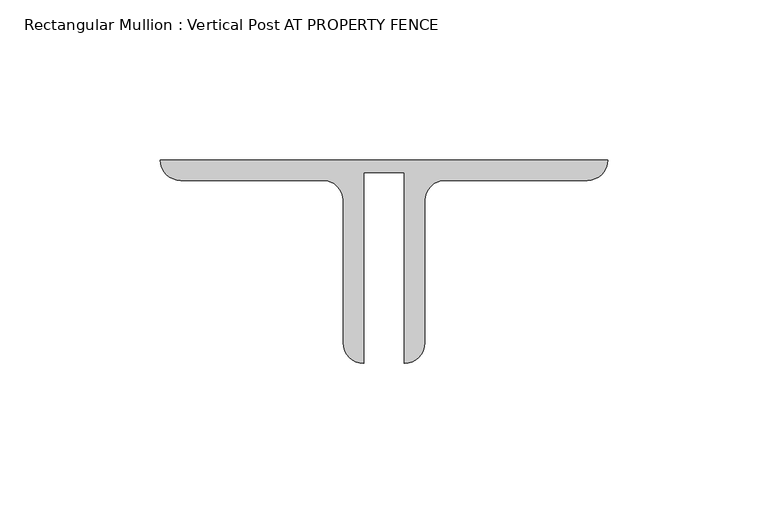
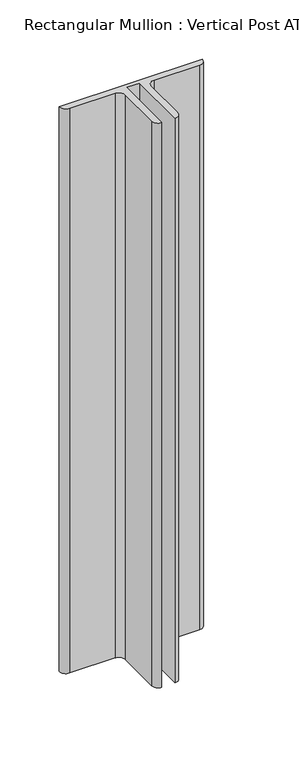
"""IFC4 building model written with IfcOpenShell, lengths in millimetres: member geometry, Rectangular Mullion : Vertical Post AT PROPERTY FENCE."""

from ifc_helpers import new_model, si_unit, point, frame, frame_2d, origin, place, context, project, spatial, polyline, circle_curve, trimmed, segment, composite_curve, outline, extrude, source, transform, mapped, element, save


def rectangular_mullion_vertical_post_at_property_fence_6001ae98(model_context):
    return source(origin(), model_context, "Body", "SweptSolid", [
        extrude(outline(composite_curve([segment(polyline([(-6.35, -22.9145205), (-6.35, -82.55)]), True, "CONTINUOUS"), segment(trimmed(circle_curve(frame_2d((-6.35, -76.2)), 6.35), [point((-6.35, -82.55))], [point((-12.7, -76.2))], False, "CARTESIAN"), True, "CONTINUOUS"), segment(polyline([(-12.7, -76.2), (-12.7, -31.75)]), True, "CONTINUOUS"), segment(trimmed(circle_curve(frame_2d((-19.05, -31.75)), 6.35), [point((-12.7, -31.75))], [point((-19.05, -25.4))], True, "CARTESIAN"), True, "CONTINUOUS"), segment(polyline([(-19.05, -25.4), (-63.5, -25.4)]), True, "CONTINUOUS"), segment(trimmed(circle_curve(frame_2d((-63.5, -19.05)), 6.35), [point((-63.5, -25.4))], [point((-69.85, -19.05))], False, "CARTESIAN"), True, "CONTINUOUS"), segment(polyline([(-69.85, -19.05), (69.85, -19.05)]), True, "CONTINUOUS"), segment(trimmed(circle_curve(frame_2d((63.5, -19.05)), 6.35), [point((69.85, -19.05))], [point((63.5, -25.4))], False, "CARTESIAN"), True, "CONTINUOUS"), segment(polyline([(63.5, -25.4), (19.05, -25.4)]), True, "CONTINUOUS"), segment(trimmed(circle_curve(frame_2d((19.05, -31.75)), 6.35), [point((19.05, -25.4))], [point((12.7, -31.75))], True, "CARTESIAN"), True, "CONTINUOUS"), segment(polyline([(12.7, -31.75), (12.7, -76.2)]), True, "CONTINUOUS"), segment(trimmed(circle_curve(frame_2d((6.35, -76.2)), 6.35), [point((12.7, -76.2))], [point((6.35, -82.55))], False, "CARTESIAN"), True, "CONTINUOUS"), segment(polyline([(6.35, -82.55), (6.35, -22.9145205), (-6.35, -22.9145205)]), True, "CONTINUOUS")], self_intersect=False)), frame((0.0, 0.0, -581.9336948), z_axis=(0.0, 0.0, 1.0), x_axis=(1.0, 0.0, 0.0)), (0.0, 0.0, 1.0), 581.9336948),
    ])


if __name__ == "__main__":
    model = new_model("IFC4")
    model_context = context("Model", 3, world=origin())
    ifc_project = project(units=[si_unit("LENGTHUNIT", "METRE", prefix="MILLI")], contexts=[model_context])
    site = spatial("IfcSite", under=ifc_project)
    building = spatial("IfcBuilding", under=site)
    placement = place(None, origin())
    rectangular_mullion_vertical_post_at_property_fence_shape = rectangular_mullion_vertical_post_at_property_fence_6001ae98(model_context)
    element("IfcMember", 1, ObjectType="Rectangular Mullion : Vertical Post AT PROPERTY FENCE", at=placement, inside=building, context=model_context, shape_type="MappedRepresentation", body=[
        mapped(rectangular_mullion_vertical_post_at_property_fence_shape, transform((0.0, 0.0, 0.0), x_axis=(1.0, 0.0, 0.0), y_axis=(0.0, 1.0, 0.0), z_axis=(0.0, 0.0, 1.0))),
    ])
    save(model, "model.ifc")

# Revit data of these elements
# Type "Rectangular Mullion : Vertical Post AT PROPERTY FENCE"
#   built-in parameter 1007351 = -0.0625 (stored number, unit not read)
#   built-in parameter 1007322 = 0.0126789 (stored number, unit not read)
#   built-in parameter 1007321 = 0.229167 (stored number, unit not read)
#   built-in parameter 1007320 = 0.229167 (stored number, unit not read)
# Element 1 (IfcMember, "Rectangular Mullion : Vertical Post AT PROPERTY FENCE")
#   Materials on its faces: "MAIN FENCE POST: (2) BACK/BACK GALVANIZED ANGLES (2) L2 1/2 X 2 1/2 X 1/4\") ANCHORED TO 8\"W X 42\" DEEP CONCRETE FOOTING(1)"
# Materials
#   "MAIN FENCE POST: (2) BACK/BACK GALVANIZED ANGLES (2) L2 1/2 X 2 1/2 X 1/4\") ANCHORED TO 8\"W X 42\" DEEP CONCRETE FOOTING(1)": class "Unassigned", colour RGB 211 211 211, transparency 0, Cost = 0
